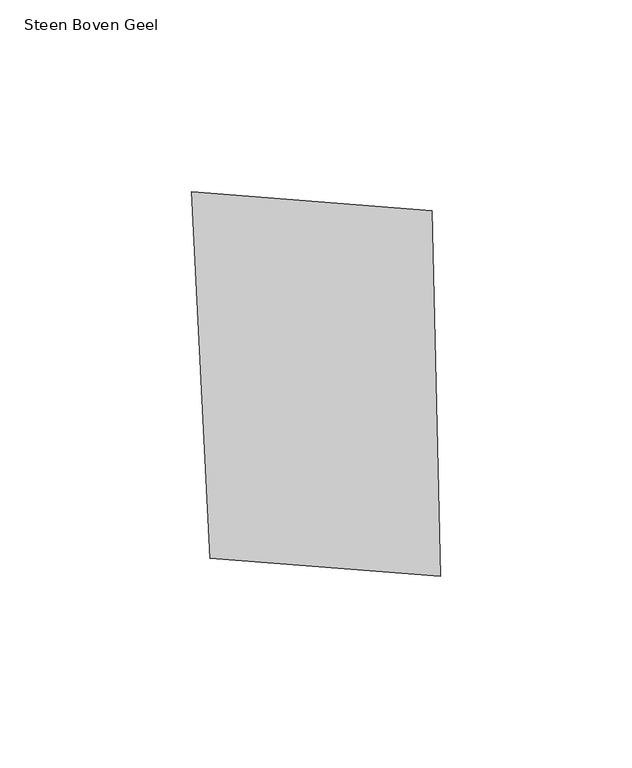
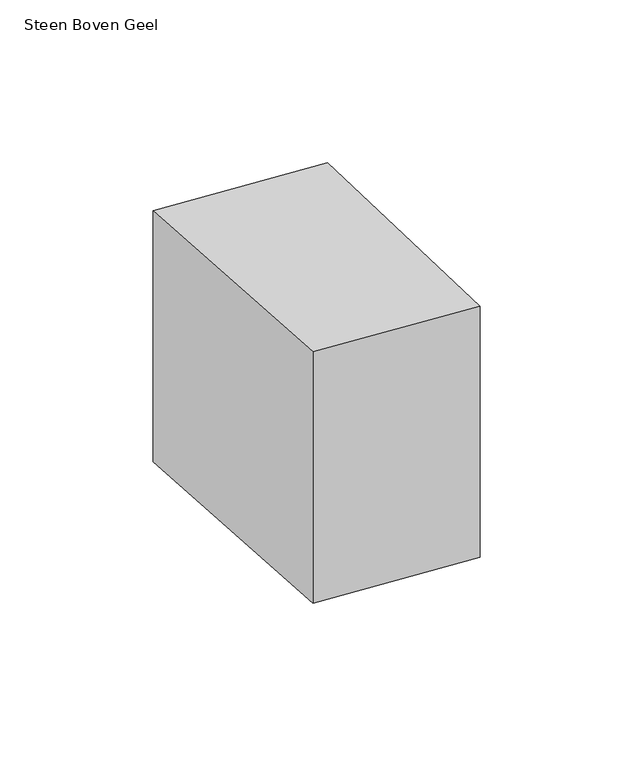
"""IFC4 building model written with IfcOpenShell, lengths in millimetres: proxy geometry, 00_GMA_steen_versie_4 : Steen Boven Geel."""

from ifc_helpers import new_model, si_unit, origin, origin_with_axes, place, context, project, spatial, polyline, outline, extrude, source, transform, mapped, element, save


def steen_boven_geel_85dfc07a(model_context):
    return source(origin(), model_context, "Body", "SweptSolid", [
        extrude(outline(polyline([(99.4214015, 119.2393918), (101.6019096, 23.7411169), (41.4923787, 28.4926929), (36.5418189, 124.2250032), (99.4214015, 119.2393918)])), origin_with_axes(), (0.0, 0.0, 1.0), 100.0),
    ])


if __name__ == "__main__":
    model = new_model("IFC4")
    model_context = context("Model", 3, world=origin())
    ifc_project = project(units=[si_unit("LENGTHUNIT", "METRE", prefix="MILLI")], contexts=[model_context])
    site = spatial("IfcSite", under=ifc_project)
    building = spatial("IfcBuilding", under=site)
    placement = place(None, origin())
    steen_boven_geel_shape = steen_boven_geel_85dfc07a(model_context)
    element("IfcBuildingElementProxy", 1, Name="00_GMA_steen_versie_4 : Steen Boven Geel", ObjectType="00_GMA_steen_versie_4 : Steen Boven Geel", at=placement, inside=building, context=model_context, shape_type="MappedRepresentation", body=[
        mapped(steen_boven_geel_shape, transform((0.0, 0.0, 0.0), x_axis=(1.0, 0.0, 0.0), y_axis=(0.0, 1.0, 0.0), z_axis=(0.0, 0.0, 1.0))),
    ])
    save(model, "model.ifc")

# Revit data of these elements
# Type "00_GMA_steen_versie_4 : Steen Boven Geel"
#   StootVoegHalfBoven [instance default] = 5 mm
#   StootVoegHalf [instance default] = 5 mm
#   StootVoegBreedteOnder = 10 mm
#   StootVoegBreedteBoven = 10 mm
#   Steendikte = 100 mm
#   LintVoegOnderHalf = 5 mm
#   LintVoegOnder = 10 mm
#   LintVoegBovenHalf = 0 mm
#   LintVoegBoven = 0 mm
#   materiaal = 21_steen_geel
#   MateriaalVoeg = none
#   Default Elevation = 0
# Element 1 (IfcBuildingElementProxy, "00_GMA_steen_versie_4 : Steen Boven Geel")
#   Materials on its faces: "21_steen_geel"
# Materials
#   "21_steen_geel": class "Unassigned", colour RGB 202 202 0, transparency 0, Cost = 0
